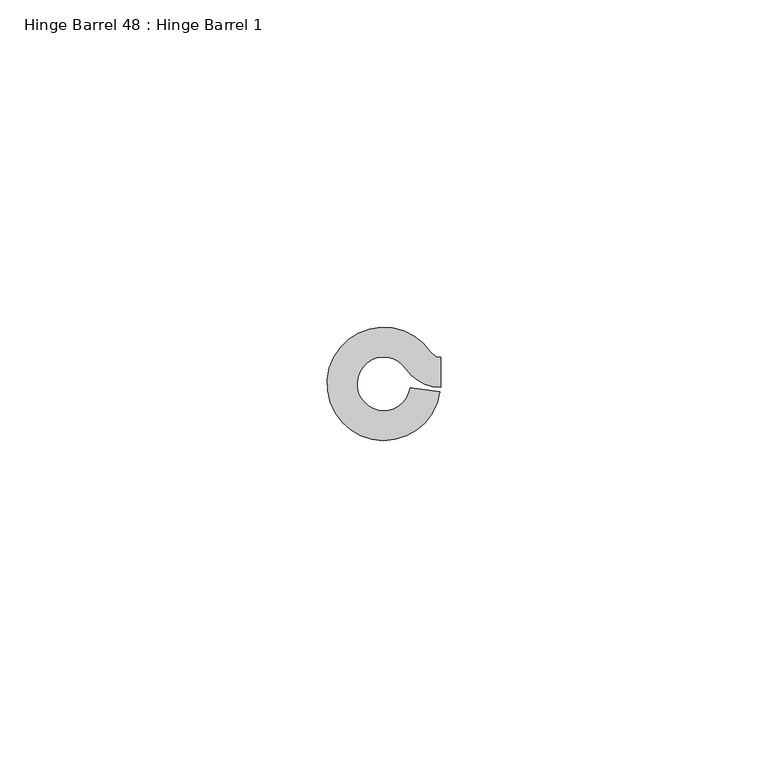
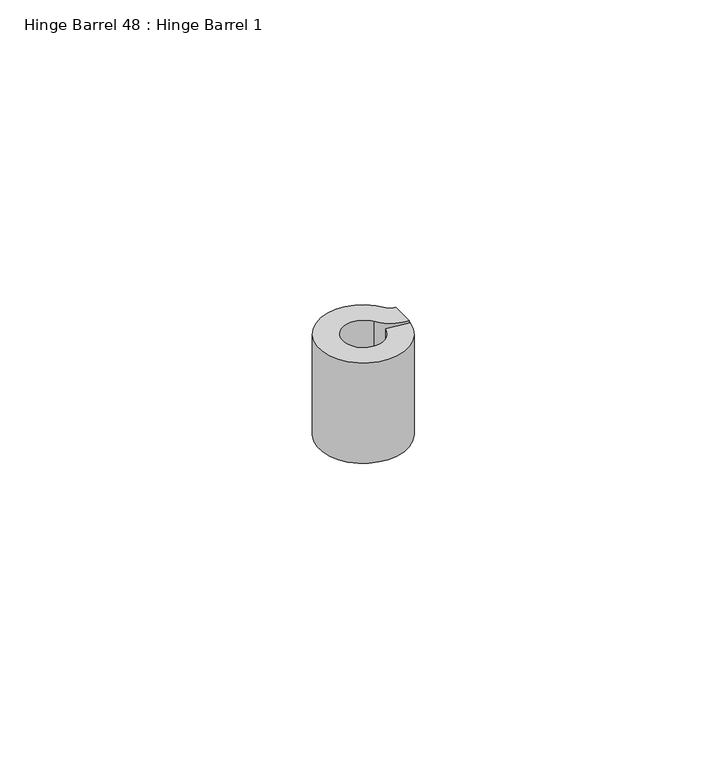
"""IFC4 building model written with IfcOpenShell, lengths in millimetres: proxy geometry, Hinge Barrel 48 : Hinge Barrel 1."""

import ifcopenshell
import ifcopenshell.guid

model = None  # the IFC model being written
_history = None  # IfcOwnerHistory: only IFC2X3 demands one
_inside = {}  # id of a spatial element -> (the spatial element, [elements in it])
_under = {}  # id of a project, library or spatial element -> (it, [spatial elements below it])
_declared = {}  # id of a project -> (the project, [libraries it declares])
_typed = {}  # id of a type object -> (the type object, [elements of that type])
_made_of = {}  # id of a material, layer set ... -> (it, [elements and type objects made of it])


def new_model(schema):
    """Start an empty IFC model of exactly this schema.

    Asked for "IFC4X3", IfcOpenShell would pick the latest addendum, in which some entities
    have other attributes; the version numbers below select the first issue.
    IFC2X3 requires an IfcOwnerHistory on every rooted entity: one is made here for all.
    """
    global model, _history
    if schema == "IFC4X3":
        model = ifcopenshell.file(schema_version=(4, 3, 0, 0))
    else:
        model = ifcopenshell.file(schema=schema)
    _inside.clear()
    _under.clear()
    _declared.clear()
    _typed.clear()
    _made_of.clear()
    _history = None
    if model.schema == "IFC2X3":
        org = make("IfcOrganization", Name="unknown")
        user = make(
            "IfcPersonAndOrganization",
            ThePerson=make("IfcPerson", FamilyName="unknown"),
            TheOrganization=org,
        )
        app = make(
            "IfcApplication",
            ApplicationDeveloper=org,
            Version="unknown",
            ApplicationFullName="unknown",
            ApplicationIdentifier="unknown",
        )
        _history = make(
            "IfcOwnerHistory",
            OwningUser=user,
            OwningApplication=app,
            ChangeAction="ADDED",
            CreationDate=0,
        )
    return model


def make(cls, **values):
    """One entity of the class cls with the attributes given. An attribute that is None is left unset."""
    return model.create_entity(
        cls, **{name: value for name, value in values.items() if value is not None}
    )


def rooted(cls, **values):
    """An entity with a GlobalId (a new one), such as an element, a storey or a relation."""
    return make(cls, GlobalId=ifcopenshell.guid.new(), OwnerHistory=_history, **values)


def si_unit(unit_type, name, prefix=None):
    """IfcSIUnit, for example si_unit("LENGTHUNIT", "METRE", prefix="MILLI")."""
    return make("IfcSIUnit", UnitType=unit_type, Prefix=prefix, Name=name)


def assignment(units):
    """IfcUnitAssignment: the units of a project."""
    return None if units is None else make("IfcUnitAssignment", Units=units)


def point(xyz):
    """IfcCartesianPoint."""
    return None if xyz is None else make("IfcCartesianPoint", Coordinates=xyz)


def direction(xyz):
    """IfcDirection."""
    return None if xyz is None else make("IfcDirection", DirectionRatios=xyz)


def frame(location, z_axis=None, x_axis=None):
    """IfcAxis2Placement3D, a coordinate frame: its origin and axes. An axis left out is left unset."""
    return make(
        "IfcAxis2Placement3D",
        Location=point(location),
        Axis=direction(z_axis),
        RefDirection=direction(x_axis),
    )


def frame_2d(location, x_axis=None):
    """IfcAxis2Placement2D, a coordinate frame in the plane: its origin and x axis."""
    return make(
        "IfcAxis2Placement2D", Location=point(location), RefDirection=direction(x_axis)
    )


def origin():
    """The frame at (0, 0, 0) with its axes left unset."""
    return frame((0.0, 0.0, 0.0))


def place(relative_to, where):
    """IfcLocalPlacement: puts the frame where relative to a parent placement (None: the world)."""
    return make(
        "IfcLocalPlacement", PlacementRelTo=relative_to, RelativePlacement=where
    )


def context(
    kind, dimensions, precision=None, world=None, true_north=None, identifier=None
):
    """IfcGeometricRepresentationContext, for example the 3D "Model" context."""
    return make(
        "IfcGeometricRepresentationContext",
        ContextIdentifier=identifier,
        ContextType=kind,
        CoordinateSpaceDimension=dimensions,
        Precision=precision,
        WorldCoordinateSystem=world,
        TrueNorth=true_north,
    )


def project(units=None, contexts=None):
    """IfcProject with its units and contexts."""
    return rooted(
        "IfcProject",
        Name="project",
        RepresentationContexts=contexts,
        UnitsInContext=assignment(units),
    )


def spatial(cls, under=None, at=None, **own):
    """A site, building, storey or space (cls), placed at a placement, below another one or the project."""
    s = rooted(cls, ObjectPlacement=at, **own)
    if under is not None:
        _under.setdefault(under.id(), (under, []))[1].append(s)
    return s


def polyline(points):
    """IfcPolyline through the points."""
    return make("IfcPolyline", Points=[point(p) for p in points])


def circle_curve(where, radius):
    """IfcCircle in the frame where."""
    return make("IfcCircle", Position=where, Radius=radius)


def trimmed(basis, trim1, trim2, sense, master):
    """IfcTrimmedCurve: the piece of a basis curve between two trims."""
    return make(
        "IfcTrimmedCurve",
        BasisCurve=basis,
        Trim1=trim1,
        Trim2=trim2,
        SenseAgreement=sense,
        MasterRepresentation=master,
    )


def segment(curve, same_sense, transition):
    """IfcCompositeCurveSegment."""
    return make(
        "IfcCompositeCurveSegment",
        Transition=transition,
        SameSense=same_sense,
        ParentCurve=curve,
    )


def composite_curve(segments, self_intersect=None):
    """IfcCompositeCurve: segments joined end to end."""
    return make("IfcCompositeCurve", Segments=segments, SelfIntersect=self_intersect)


def outline(outer, holes=None, kind="AREA"):
    """IfcArbitraryClosedProfileDef: a profile drawn as a closed curve; with holes, ...WithVoids."""
    if holes is None:
        return make("IfcArbitraryClosedProfileDef", ProfileType=kind, OuterCurve=outer)
    return make(
        "IfcArbitraryProfileDefWithVoids",
        ProfileType=kind,
        OuterCurve=outer,
        InnerCurves=holes,
    )


def extrude(swept, where, along, depth):
    """IfcExtrudedAreaSolid: the profile swept, set in the frame where, extruded along a direction by depth."""
    return make(
        "IfcExtrudedAreaSolid",
        SweptArea=swept,
        Position=where,
        ExtrudedDirection=direction(along),
        Depth=depth,
    )


def shape(context_of_items, identifier, shape_type, items):
    """IfcShapeRepresentation: the items that make up one representation, for example the "Body"."""
    return make(
        "IfcShapeRepresentation",
        ContextOfItems=context_of_items,
        RepresentationIdentifier=identifier,
        RepresentationType=shape_type,
        Items=items,
    )


def source(mapping_origin, context_of_items, identifier, shape_type, items):
    """IfcRepresentationMap: a shape defined once, which mapped items show again and again."""
    return make(
        "IfcRepresentationMap",
        MappingOrigin=mapping_origin,
        MappedRepresentation=shape(context_of_items, identifier, shape_type, items),
    )


def transform(
    local_origin,
    x_axis=None,
    y_axis=None,
    z_axis=None,
    scale=None,
    scale2=None,
    scale3=None,
    uniform=True,
):
    """IfcCartesianTransformationOperator3D, or its non-uniform kind. x_axis, y_axis, z_axis: its Axis1, 2, 3."""
    if uniform:
        return make(
            "IfcCartesianTransformationOperator3D",
            Axis1=direction(x_axis),
            Axis2=direction(y_axis),
            LocalOrigin=point(local_origin),
            Scale=scale,
            Axis3=direction(z_axis),
        )
    return make(
        "IfcCartesianTransformationOperator3DnonUniform",
        Axis1=direction(x_axis),
        Axis2=direction(y_axis),
        LocalOrigin=point(local_origin),
        Scale=scale,
        Axis3=direction(z_axis),
        Scale2=scale2,
        Scale3=scale3,
    )


def mapped(mapping_source, mapping_target):
    """IfcMappedItem: shows the shape of a source again, moved by a transform."""
    return make(
        "IfcMappedItem", MappingSource=mapping_source, MappingTarget=mapping_target
    )


def made_of(thing, what):
    """Note that an element or type object is made of a material, layer set ...; save() writes the relation."""
    if what is not None:
        _made_of.setdefault(what.id(), (what, []))[1].append(thing)
    return thing


def element(
    cls,
    number,
    at=None,
    inside=None,
    cuts=None,
    type_object=None,
    material=None,
    context=None,
    identifier="Body",
    shape_type=None,
    held_by="IfcProductDefinitionShape",
    body=None,
    shapes=None,
    **own,
):
    """One element of the class cls, such as IfcWall. Its Tag is "e" and its number.

    at: its placement. inside: the storey or other place that contains it. cuts: it is an
    opening in that element (IfcRelVoidsElement). A single representation is given by context,
    identifier, shape_type and body (its items); several are given by shapes. held_by: the class
    of the entity that holds the representations. save() writes the other relations.
    """
    e = rooted(cls, Tag="e%d" % number, ObjectPlacement=at, **own)
    if body is not None:
        shapes = [shape(context, identifier, shape_type, body)]
    if shapes is not None:
        e.Representation = make(held_by, Representations=shapes)
    if inside is not None:
        _inside.setdefault(inside.id(), (inside, []))[1].append(e)
    if cuts is not None:
        rooted(
            "IfcRelVoidsElement", RelatingBuildingElement=cuts, RelatedOpeningElement=e
        )
    if type_object is not None:
        _typed.setdefault(type_object.id(), (type_object, []))[1].append(e)
    return made_of(e, material)


def aggregate(whole, parts):
    """IfcRelAggregates: a whole, such as a stair, and the parts it consists of."""
    return rooted("IfcRelAggregates", RelatingObject=whole, RelatedObjects=parts)


def save(model, path):
    """Write the relations noted so far, then the file.

    IfcRelAggregates (storeys below a building ...), IfcRelContainedInSpatialStructure (elements
    in a storey), IfcRelDefinesByType, IfcRelAssociatesMaterial and IfcRelDeclares: one each for
    every whole, place, type object, material and project.
    """
    for whole, parts in _under.values():
        aggregate(whole, parts)
    for where, things in _inside.values():
        rooted(
            "IfcRelContainedInSpatialStructure",
            RelatedElements=things,
            RelatingStructure=where,
        )
    for kind, things in _typed.values():
        rooted("IfcRelDefinesByType", RelatedObjects=things, RelatingType=kind)
    for what, things in _made_of.values():
        rooted("IfcRelAssociatesMaterial", RelatedObjects=things, RelatingMaterial=what)
    for by, libraries in _declared.values():
        rooted("IfcRelDeclares", RelatingContext=by, RelatedDefinitions=libraries)
    model.write(path)


def hinge_barrel_48_hinge_barrel_1_1e94fffa(model_context):
    return source(origin(), model_context, "Body", "SweptSolid", [
        extrude(outline(composite_curve([segment(trimmed(circle_curve(frame_2d((587319.1320739, -534100.7049841)), 4.0894), [point((587322.5194669, -534098.4139665))], [point((587323.1821338, -534101.2708529))], True, "CARTESIAN"), True, "CONTINUOUS"), segment(polyline([(587323.1821338, -534101.2708529), (587327.7022899, -534101.9024028)]), True, "CONTINUOUS"), segment(trimmed(circle_curve(frame_2d((587319.1320739, -534100.7049841)), 8.6534625), [point((587327.7022899, -534101.9024028))], [point((587326.3000393, -534095.8570273))], False, "CARTESIAN"), True, "CONTINUOUS"), segment(trimmed(circle_curve(frame_2d((587327.8245257, -534094.8259615)), 1.8404226), [point((587326.3000393, -534095.8570273))], [point((587327.8245257, -534096.6663841))], True, "CARTESIAN"), True, "CONTINUOUS"), segment(polyline([(587327.8245257, -534096.6663841), (587327.8245257, -534101.2304466)]), True, "CONTINUOUS"), segment(trimmed(circle_curve(frame_2d((587327.8245257, -534094.8259615)), 6.4044851), [point((587327.8245257, -534101.2304466))], [point((587322.5194669, -534098.4139665))], False, "CARTESIAN"), True, "CONTINUOUS")], self_intersect=False)), frame((0.0, 0.0, 2063.75), z_axis=(0.0, 0.0, 1.0), x_axis=(1.0, 0.0, 0.0)), (0.0, 0.0, 1.0), 20.8359375),
    ])


if __name__ == "__main__":
    model = new_model("IFC4")
    model_context = context("Model", 3, world=origin())
    ifc_project = project(units=[si_unit("LENGTHUNIT", "METRE", prefix="MILLI")], contexts=[model_context])
    site = spatial("IfcSite", under=ifc_project)
    building = spatial("IfcBuilding", under=site)
    placement = place(None, origin())
    hinge_barrel_48_hinge_barrel_1_shape = hinge_barrel_48_hinge_barrel_1_1e94fffa(model_context)
    element("IfcBuildingElementProxy", 1, Name="Hinge Barrel 48 : Hinge Barrel 1", ObjectType="Hinge Barrel 48 : Hinge Barrel 1", at=placement, inside=building, context=model_context, shape_type="MappedRepresentation", body=[
        mapped(hinge_barrel_48_hinge_barrel_1_shape, transform((0.0, 0.0, 0.0), x_axis=(1.0, 0.0, 0.0), y_axis=(0.0, 1.0, 0.0), z_axis=(0.0, 0.0, 1.0))),
    ])
    save(model, "model.ifc")

# Revit data of these elements
# Element 1 (IfcBuildingElementProxy, "Hinge Barrel 48 : Hinge Barrel 1")
#   Materials on its faces: "6\"X6\" WELD-ON STL BUTT HINGE"
# Materials
#   "6\"X6\" WELD-ON STL BUTT HINGE": class "Metal", colour RGB 189 187 185, transparency 0, Description = "Carbon steel", Cost = 0
